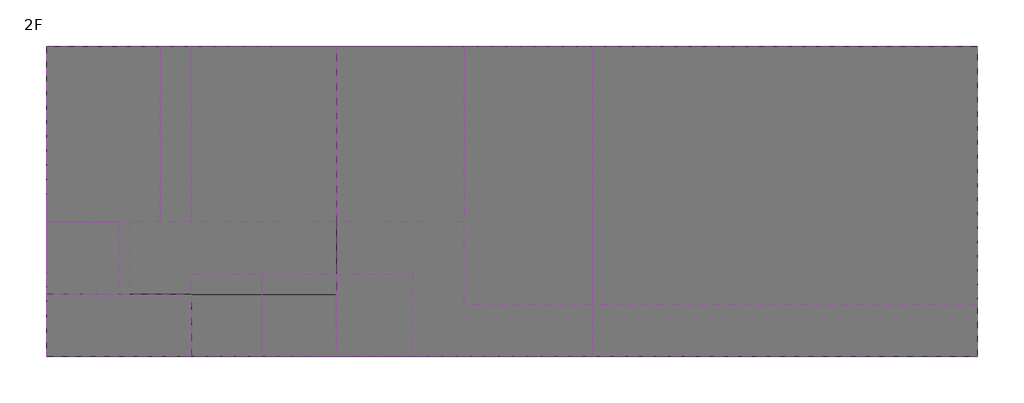
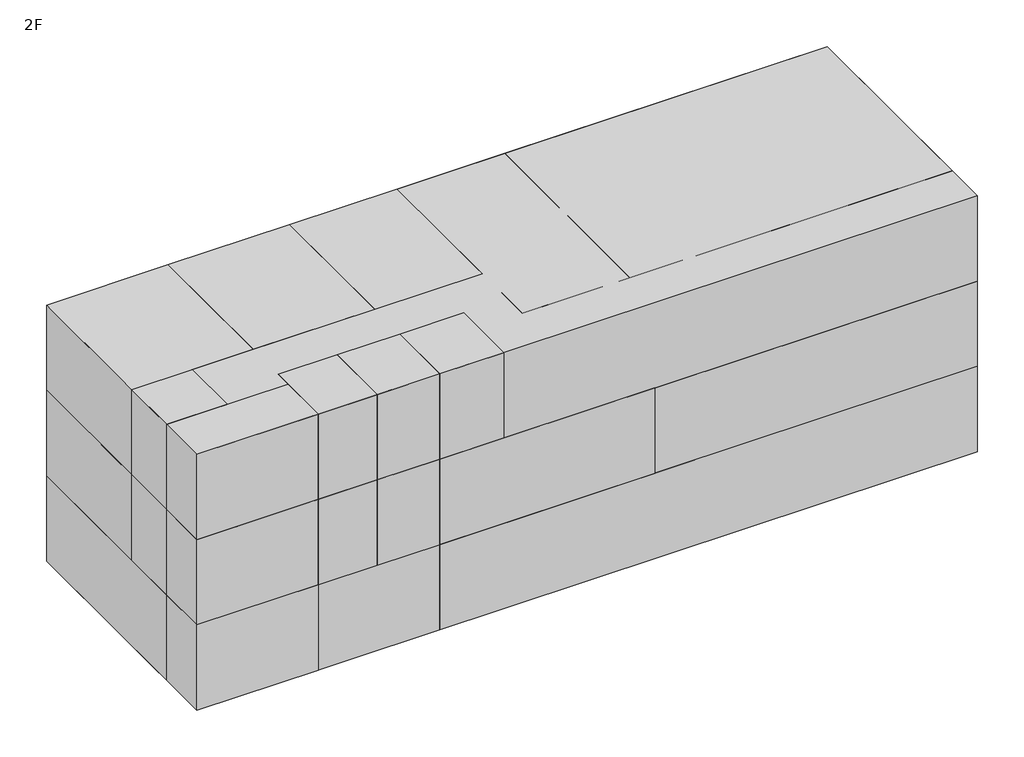
# One storey: 24 proxies.
"""IFC4 building model written with IfcOpenShell, lengths in millimetres."""

import ifcopenshell
import ifcopenshell.guid

model = None  # the IFC model being written
_history = None  # IfcOwnerHistory: only IFC2X3 demands one
_inside = {}  # id of a spatial element -> (the spatial element, [elements in it])
_under = {}  # id of a project, library or spatial element -> (it, [spatial elements below it])
_declared = {}  # id of a project -> (the project, [libraries it declares])
_typed = {}  # id of a type object -> (the type object, [elements of that type])
_made_of = {}  # id of a material, layer set ... -> (it, [elements and type objects made of it])


def new_model(schema):
    """Start an empty IFC model of exactly this schema.

    Asked for "IFC4X3", IfcOpenShell would pick the latest addendum, in which some entities
    have other attributes; the version numbers below select the first issue.
    IFC2X3 requires an IfcOwnerHistory on every rooted entity: one is made here for all.
    """
    global model, _history
    if schema == "IFC4X3":
        model = ifcopenshell.file(schema_version=(4, 3, 0, 0))
    else:
        model = ifcopenshell.file(schema=schema)
    _inside.clear()
    _under.clear()
    _declared.clear()
    _typed.clear()
    _made_of.clear()
    _history = None
    if model.schema == "IFC2X3":
        org = make("IfcOrganization", Name="unknown")
        user = make(
            "IfcPersonAndOrganization",
            ThePerson=make("IfcPerson", FamilyName="unknown"),
            TheOrganization=org,
        )
        app = make(
            "IfcApplication",
            ApplicationDeveloper=org,
            Version="unknown",
            ApplicationFullName="unknown",
            ApplicationIdentifier="unknown",
        )
        _history = make(
            "IfcOwnerHistory",
            OwningUser=user,
            OwningApplication=app,
            ChangeAction="ADDED",
            CreationDate=0,
        )
    return model


def make(cls, **values):
    """One entity of the class cls with the attributes given. An attribute that is None is left unset."""
    return model.create_entity(
        cls, **{name: value for name, value in values.items() if value is not None}
    )


def rooted(cls, **values):
    """An entity with a GlobalId (a new one), such as an element, a storey or a relation."""
    return make(cls, GlobalId=ifcopenshell.guid.new(), OwnerHistory=_history, **values)


def si_unit(unit_type, name, prefix=None):
    """IfcSIUnit, for example si_unit("LENGTHUNIT", "METRE", prefix="MILLI")."""
    return make("IfcSIUnit", UnitType=unit_type, Prefix=prefix, Name=name)


def assignment(units):
    """IfcUnitAssignment: the units of a project."""
    return None if units is None else make("IfcUnitAssignment", Units=units)


def point(xyz):
    """IfcCartesianPoint."""
    return None if xyz is None else make("IfcCartesianPoint", Coordinates=xyz)


def direction(xyz):
    """IfcDirection."""
    return None if xyz is None else make("IfcDirection", DirectionRatios=xyz)


def frame(location, z_axis=None, x_axis=None):
    """IfcAxis2Placement3D, a coordinate frame: its origin and axes. An axis left out is left unset."""
    return make(
        "IfcAxis2Placement3D",
        Location=point(location),
        Axis=direction(z_axis),
        RefDirection=direction(x_axis),
    )


def origin():
    """The frame at (0, 0, 0) with its axes left unset."""
    return frame((0.0, 0.0, 0.0))


def origin_with_axes():
    """The frame at (0, 0, 0) with the z axis (0, 0, 1) and the x axis (1, 0, 0) written out."""
    return frame((0.0, 0.0, 0.0), z_axis=(0.0, 0.0, 1.0), x_axis=(1.0, 0.0, 0.0))


def place(relative_to, where):
    """IfcLocalPlacement: puts the frame where relative to a parent placement (None: the world)."""
    return make(
        "IfcLocalPlacement", PlacementRelTo=relative_to, RelativePlacement=where
    )


def context(
    kind, dimensions, precision=None, world=None, true_north=None, identifier=None
):
    """IfcGeometricRepresentationContext, for example the 3D "Model" context."""
    return make(
        "IfcGeometricRepresentationContext",
        ContextIdentifier=identifier,
        ContextType=kind,
        CoordinateSpaceDimension=dimensions,
        Precision=precision,
        WorldCoordinateSystem=world,
        TrueNorth=true_north,
    )


def project(units=None, contexts=None):
    """IfcProject with its units and contexts."""
    return rooted(
        "IfcProject",
        Name="project",
        RepresentationContexts=contexts,
        UnitsInContext=assignment(units),
    )


def spatial(cls, under=None, at=None, **own):
    """A site, building, storey or space (cls), placed at a placement, below another one or the project."""
    s = rooted(cls, ObjectPlacement=at, **own)
    if under is not None:
        _under.setdefault(under.id(), (under, []))[1].append(s)
    return s


def polyline(points):
    """IfcPolyline through the points."""
    return make("IfcPolyline", Points=[point(p) for p in points])


def outline(outer, holes=None, kind="AREA"):
    """IfcArbitraryClosedProfileDef: a profile drawn as a closed curve; with holes, ...WithVoids."""
    if holes is None:
        return make("IfcArbitraryClosedProfileDef", ProfileType=kind, OuterCurve=outer)
    return make(
        "IfcArbitraryProfileDefWithVoids",
        ProfileType=kind,
        OuterCurve=outer,
        InnerCurves=holes,
    )


def extrude(swept, where, along, depth):
    """IfcExtrudedAreaSolid: the profile swept, set in the frame where, extruded along a direction by depth."""
    return make(
        "IfcExtrudedAreaSolid",
        SweptArea=swept,
        Position=where,
        ExtrudedDirection=direction(along),
        Depth=depth,
    )


def shape(context_of_items, identifier, shape_type, items):
    """IfcShapeRepresentation: the items that make up one representation, for example the "Body"."""
    return make(
        "IfcShapeRepresentation",
        ContextOfItems=context_of_items,
        RepresentationIdentifier=identifier,
        RepresentationType=shape_type,
        Items=items,
    )


def source(mapping_origin, context_of_items, identifier, shape_type, items):
    """IfcRepresentationMap: a shape defined once, which mapped items show again and again."""
    return make(
        "IfcRepresentationMap",
        MappingOrigin=mapping_origin,
        MappedRepresentation=shape(context_of_items, identifier, shape_type, items),
    )


def transform(
    local_origin,
    x_axis=None,
    y_axis=None,
    z_axis=None,
    scale=None,
    scale2=None,
    scale3=None,
    uniform=True,
):
    """IfcCartesianTransformationOperator3D, or its non-uniform kind. x_axis, y_axis, z_axis: its Axis1, 2, 3."""
    if uniform:
        return make(
            "IfcCartesianTransformationOperator3D",
            Axis1=direction(x_axis),
            Axis2=direction(y_axis),
            LocalOrigin=point(local_origin),
            Scale=scale,
            Axis3=direction(z_axis),
        )
    return make(
        "IfcCartesianTransformationOperator3DnonUniform",
        Axis1=direction(x_axis),
        Axis2=direction(y_axis),
        LocalOrigin=point(local_origin),
        Scale=scale,
        Axis3=direction(z_axis),
        Scale2=scale2,
        Scale3=scale3,
    )


def mapped(mapping_source, mapping_target):
    """IfcMappedItem: shows the shape of a source again, moved by a transform."""
    return make(
        "IfcMappedItem", MappingSource=mapping_source, MappingTarget=mapping_target
    )


def made_of(thing, what):
    """Note that an element or type object is made of a material, layer set ...; save() writes the relation."""
    if what is not None:
        _made_of.setdefault(what.id(), (what, []))[1].append(thing)
    return thing


def element(
    cls,
    number,
    at=None,
    inside=None,
    cuts=None,
    type_object=None,
    material=None,
    context=None,
    identifier="Body",
    shape_type=None,
    held_by="IfcProductDefinitionShape",
    body=None,
    shapes=None,
    **own,
):
    """One element of the class cls, such as IfcWall. Its Tag is "e" and its number.

    at: its placement. inside: the storey or other place that contains it. cuts: it is an
    opening in that element (IfcRelVoidsElement). A single representation is given by context,
    identifier, shape_type and body (its items); several are given by shapes. held_by: the class
    of the entity that holds the representations. save() writes the other relations.
    """
    e = rooted(cls, Tag="e%d" % number, ObjectPlacement=at, **own)
    if body is not None:
        shapes = [shape(context, identifier, shape_type, body)]
    if shapes is not None:
        e.Representation = make(held_by, Representations=shapes)
    if inside is not None:
        _inside.setdefault(inside.id(), (inside, []))[1].append(e)
    if cuts is not None:
        rooted(
            "IfcRelVoidsElement", RelatingBuildingElement=cuts, RelatedOpeningElement=e
        )
    if type_object is not None:
        _typed.setdefault(type_object.id(), (type_object, []))[1].append(e)
    return made_of(e, material)


def aggregate(whole, parts):
    """IfcRelAggregates: a whole, such as a stair, and the parts it consists of."""
    return rooted("IfcRelAggregates", RelatingObject=whole, RelatedObjects=parts)


def save(model, path):
    """Write the relations noted so far, then the file.

    IfcRelAggregates (storeys below a building ...), IfcRelContainedInSpatialStructure (elements
    in a storey), IfcRelDefinesByType, IfcRelAssociatesMaterial and IfcRelDeclares: one each for
    every whole, place, type object, material and project.
    """
    for whole, parts in _under.values():
        aggregate(whole, parts)
    for where, things in _inside.values():
        rooted(
            "IfcRelContainedInSpatialStructure",
            RelatedElements=things,
            RelatingStructure=where,
        )
    for kind, things in _typed.values():
        rooted("IfcRelDefinesByType", RelatedObjects=things, RelatingType=kind)
    for what, things in _made_of.values():
        rooted("IfcRelAssociatesMaterial", RelatedObjects=things, RelatingMaterial=what)
    for by, libraries in _declared.values():
        rooted("IfcRelDeclares", RelatingContext=by, RelatedDefinitions=libraries)
    model.write(path)


def generic_models_32ca781f(model_context):
    return source(origin(), model_context, "Body", "SweptSolid", [
        extrude(outline(polyline([(15500.0, 7500.0), (15500.0, -7500.0), (-15500.0, -7500.0), (-15500.0, 7500.0), (15500.0, 7500.0)])), origin_with_axes(), (0.0, 0.0, 1.0), 5200.0),
    ])


def generic_models_ec4f78ea(model_context):
    return source(origin(), model_context, "Body", "SweptSolid", [
        extrude(outline(polyline([(7000.0, 6000.0), (7000.0, -6000.0), (-7000.0, -6000.0), (-7000.0, 6000.0), (7000.0, 6000.0)])), origin_with_axes(), (0.0, 0.0, 1.0), 5200.0),
    ])


def generic_models_2e4aee51(model_context):
    return source(origin(), model_context, "Body", "SweptSolid", [
        extrude(outline(polyline([(1500.0, 3500.0), (1500.0, -3500.0), (-1500.0, -3500.0), (-1500.0, 3500.0), (1500.0, 3500.0)])), origin_with_axes(), (0.0, 0.0, 1.0), 5200.0),
    ])


def generic_models_246d78d5(model_context):
    return source(origin(), model_context, "Body", "SweptSolid", [
        extrude(outline(polyline([(6200.0, 7500.0), (6200.0, -7500.0), (-6200.0, -7500.0), (-6200.0, 7500.0), (6200.0, 7500.0)])), origin_with_axes(), (0.0, 0.0, 1.0), 5200.0),
    ])


def generic_models_5fb19e15(model_context):
    return source(origin(), model_context, "Body", "SweptSolid", [
        extrude(outline(polyline([(9300.0, 7500.0), (9300.0, -7500.0), (-9300.0, -7500.0), (-9300.0, 7500.0), (9300.0, 7500.0)])), origin_with_axes(), (0.0, 0.0, 1.0), 5200.0),
    ])


def generic_models_c4e3d020(model_context):
    return source(origin(), model_context, "Body", "SweptSolid", [
        extrude(outline(polyline([(4250.0, 4250.0), (4250.0, -4250.0), (-4250.0, -4250.0), (-4250.0, 4250.0), (4250.0, 4250.0)])), origin_with_axes(), (0.0, 0.0, 1.0), 5200.0),
    ])


def generic_models_d0c3260c(model_context):
    return source(origin(), model_context, "Body", "SweptSolid", [
        extrude(outline(polyline([(2750.0, 4250.0), (2750.0, -4250.0), (-2750.0, -4250.0), (-2750.0, 4250.0), (2750.0, 4250.0)])), origin_with_axes(), (0.0, 0.0, 1.0), 5200.0),
    ])


def generic_models_2b76ab57(model_context):
    return source(origin(), model_context, "Body", "SweptSolid", [
        extrude(outline(polyline([(1800.0, 2000.0), (1800.0, -2000.0), (-1800.0, -2000.0), (-1800.0, 2000.0), (1800.0, 2000.0)])), origin_with_axes(), (0.0, 0.0, 1.0), 5200.0),
    ])


def generic_models_5d679b5e(model_context):
    return source(origin(), model_context, "Body", "SweptSolid", [
        extrude(outline(polyline([(1700.0, 2000.0), (1700.0, -2000.0), (-1700.0, -2000.0), (-1700.0, 2000.0), (1700.0, 2000.0)])), origin_with_axes(), (0.0, 0.0, 1.0), 5200.0),
    ])


def generic_models_7d267c0d(model_context):
    return source(origin(), model_context, "Body", "SweptSolid", [
        extrude(outline(polyline([(1750.0, 2000.0), (1750.0, -2000.0), (-1750.0, -2000.0), (-1750.0, 2000.0), (1750.0, 2000.0)])), origin_with_axes(), (0.0, 0.0, 1.0), 5200.0),
    ])


def generic_models_235df1fa(model_context):
    return source(origin(), model_context, "Body", "SweptSolid", [
        extrude(outline(polyline([(3500.0, 4250.0), (3500.0, -4250.0), (-3500.0, -4250.0), (-3500.0, 4250.0), (3500.0, 4250.0)])), origin_with_axes(), (0.0, 0.0, 1.0), 5200.0),
    ])


def generic_models_228d8ca4(model_context):
    return source(origin(), model_context, "Body", "SweptSolid", [
        extrude(outline(polyline([(3100.0, 4250.0), (3100.0, -4250.0), (-3100.0, -4250.0), (-3100.0, 4250.0), (3100.0, 4250.0)])), origin_with_axes(), (0.0, 0.0, 1.0), 5200.0),
    ])


def generic_models_f38cfd17(model_context):
    return source(origin(), model_context, "Body", "SweptSolid", [
        extrude(outline(polyline([(3100.0, 6250.0), (3100.0, -6250.0), (-3100.0, -6250.0), (-3100.0, 6250.0), (3100.0, 6250.0)])), origin_with_axes(), (0.0, 0.0, 1.0), 5200.0),
    ])


def generic_models_0e92175d(model_context):
    return source(origin(), model_context, "Body", "SweptSolid", [
        extrude(outline(polyline([(2000.0, 1850.0), (2000.0, -1850.0), (-2000.0, -1850.0), (-2000.0, 1850.0), (2000.0, 1850.0)])), origin_with_axes(), (0.0, 0.0, 1.0), 5200.0),
    ])


def generic_models_412ad42b(model_context):
    return source(origin(), model_context, "Body", "SweptSolid", [
        extrude(outline(polyline([(1750.0, 1750.0), (1750.0, -1750.0), (-1750.0, -1750.0), (-1750.0, 1750.0), (1750.0, 1750.0)])), origin_with_axes(), (0.0, 0.0, 1.0), 5200.0),
    ])


def generic_models_608d95d2(model_context):
    return source(origin(), model_context, "Body", "SweptSolid", [
        extrude(outline(polyline([(9300.0, 6250.0), (9300.0, -6250.0), (-9300.0, -6250.0), (-9300.0, 6250.0), (9300.0, 6250.0)])), origin_with_axes(), (0.0, 0.0, 1.0), 5200.0),
    ])


def generic_models_083cc7c1(model_context):
    return source(origin(), model_context, "Body", "SweptSolid", [
        extrude(outline(polyline([(7500.0, 22500.0), (7500.0, -22500.0), (-7500.0, -22500.0), (-7500.0, 22500.0), (7500.0, 22500.0)])), origin_with_axes(), (0.0, 0.0, 1.0), 5200.0),
    ])


model = new_model("IFC4")

# Units and contexts
model_context = context("Model", 3, world=origin())
ifc_project = project(units=[si_unit("LENGTHUNIT", "METRE", prefix="MILLI")], contexts=[model_context])

# Site, building, storey
site = spatial("IfcSite", under=ifc_project)
building = spatial("IfcBuilding", under=site)
storey = spatial("IfcBuildingStorey", under=building, Name="2F", Elevation=5500.0)

# Proxies
placement = place(None, origin())
generic_models_shape = generic_models_32ca781f(model_context)
element("IfcBuildingElementProxy", 1, Name="Space Planning Box_hec : Space Planning Box_hec", ObjectType="Space Planning Box_hec : Space Planning Box_hec", at=placement, inside=storey, context=model_context, shape_type="MappedRepresentation", body=[
    mapped(generic_models_shape, transform((74959.6521483, 179923.8614395, 5500.0), x_axis=(1.0, 0.0, 0.0), y_axis=(0.0, 1.0, 0.0), z_axis=(0.0, 0.0, 1.0))),
])
generic_models_2_shape = generic_models_ec4f78ea(model_context)
element("IfcBuildingElementProxy", 2, Name="Space Planning Box_hec : Space Planning Box_hec", ObjectType="Space Planning Box_hec : Space Planning Box_hec", at=placement, inside=storey, context=model_context, shape_type="MappedRepresentation", body=[
    mapped(generic_models_2_shape, transform((52459.6521483, 181423.8614395, 5500.0), x_axis=(1.0, 0.0, 0.0), y_axis=(0.0, 1.0, 0.0), z_axis=(0.0, 0.0, 1.0))),
])
generic_models_3_shape = generic_models_2e4aee51(model_context)
element("IfcBuildingElementProxy", 3, Name="Space Planning Box_hec : Space Planning Box_hec", ObjectType="Space Planning Box_hec : Space Planning Box_hec", at=placement, inside=storey, context=model_context, shape_type="MappedRepresentation", body=[
    mapped(generic_models_3_shape, transform((48959.6521483, 173923.8614395, 5500.0), x_axis=(0.0, 1.0, 0.0), y_axis=(-1.0, 0.0, 0.0), z_axis=(0.0, 0.0, 1.0))),
])
element("IfcBuildingElementProxy", 4, Name="Space Planning Box_hec : Space Planning Box_hec", ObjectType="Space Planning Box_hec : Space Planning Box_hec", at=placement, inside=storey, context=model_context, shape_type="MappedRepresentation", body=[
    mapped(generic_models_3_shape, transform((48959.6521483, 173923.8614395, 10700.0), x_axis=(0.0, 1.0, 0.0), y_axis=(-1.0, 0.0, 0.0), z_axis=(0.0, 0.0, 1.0))),
])
element("IfcBuildingElementProxy", 5, Name="Space Planning Box_hec : Space Planning Box_hec", ObjectType="Space Planning Box_hec : Space Planning Box_hec", at=placement, inside=storey, context=model_context, shape_type="MappedRepresentation", body=[
    mapped(generic_models_3_shape, transform((48959.6521483, 173923.8614395, 15900.0), x_axis=(0.0, 1.0, 0.0), y_axis=(-1.0, 0.0, 0.0), z_axis=(0.0, 0.0, 1.0))),
])
generic_models_4_shape = generic_models_246d78d5(model_context)
element("IfcBuildingElementProxy", 6, Name="Space Planning Box_hec : Space Planning Box_hec", ObjectType="Space Planning Box_hec : Space Planning Box_hec", at=placement, inside=storey, context=model_context, shape_type="MappedRepresentation", body=[
    mapped(generic_models_4_shape, transform((65659.6521483, 179923.8614395, 10700.0), x_axis=(1.0, 0.0, 0.0), y_axis=(0.0, 1.0, 0.0), z_axis=(0.0, 0.0, 1.0))),
])
generic_models_5_shape = generic_models_5fb19e15(model_context)
element("IfcBuildingElementProxy", 7, Name="Space Planning Box_hec : Space Planning Box_hec", ObjectType="Space Planning Box_hec : Space Planning Box_hec", at=placement, inside=storey, context=model_context, shape_type="MappedRepresentation", body=[
    mapped(generic_models_5_shape, transform((81159.6521483, 179923.8614395, 10700.0), x_axis=(1.0, 0.0, 0.0), y_axis=(0.0, 1.0, 0.0), z_axis=(0.0, 0.0, 1.0))),
])
generic_models_6_shape = generic_models_c4e3d020(model_context)
element("IfcBuildingElementProxy", 8, Name="Space Planning Box_hec : Space Planning Box_hec", ObjectType="Space Planning Box_hec : Space Planning Box_hec", at=placement, inside=storey, context=model_context, shape_type="MappedRepresentation", body=[
    mapped(generic_models_6_shape, transform((55209.6521483, 183173.8614395, 10700.0), x_axis=(-1.0, 0.0, 0.0), y_axis=(0.0, -1.0, 0.0), z_axis=(0.0, 0.0, 1.0))),
])
generic_models_7_shape = generic_models_d0c3260c(model_context)
element("IfcBuildingElementProxy", 9, Name="Space Planning Box_hec : Space Planning Box_hec", ObjectType="Space Planning Box_hec : Space Planning Box_hec", at=placement, inside=storey, context=model_context, shape_type="MappedRepresentation", body=[
    mapped(generic_models_7_shape, transform((48209.6521483, 183173.8614395, 10700.0), x_axis=(1.0, 0.0, 0.0), y_axis=(0.0, 1.0, 0.0), z_axis=(0.0, 0.0, 1.0))),
])
generic_models_8_shape = generic_models_2b76ab57(model_context)
element("IfcBuildingElementProxy", 10, Name="Space Planning Box_hec : Space Planning Box_hec", ObjectType="Space Planning Box_hec : Space Planning Box_hec", at=placement, inside=storey, context=model_context, shape_type="MappedRepresentation", body=[
    mapped(generic_models_8_shape, transform((57659.6521483, 174423.8614395, 10700.0), x_axis=(1.0, 0.0, 0.0), y_axis=(0.0, 1.0, 0.0), z_axis=(0.0, 0.0, 1.0))),
])
element("IfcBuildingElementProxy", 11, Name="Space Planning Box_hec : Space Planning Box_hec", ObjectType="Space Planning Box_hec : Space Planning Box_hec", at=placement, inside=storey, context=model_context, shape_type="MappedRepresentation", body=[
    mapped(generic_models_8_shape, transform((57659.6521483, 174423.8614395, 15900.0), x_axis=(1.0, 0.0, 0.0), y_axis=(0.0, 1.0, 0.0), z_axis=(0.0, 0.0, 1.0))),
])
generic_models_9_shape = generic_models_5d679b5e(model_context)
element("IfcBuildingElementProxy", 12, Name="Space Planning Box_hec : Space Planning Box_hec", ObjectType="Space Planning Box_hec : Space Planning Box_hec", at=placement, inside=storey, context=model_context, shape_type="MappedRepresentation", body=[
    mapped(generic_models_9_shape, transform((54159.6521483, 174423.8614395, 10700.0), x_axis=(1.0, 0.0, 0.0), y_axis=(0.0, 1.0, 0.0), z_axis=(0.0, 0.0, 1.0))),
])
element("IfcBuildingElementProxy", 13, Name="Space Planning Box_hec : Space Planning Box_hec", ObjectType="Space Planning Box_hec : Space Planning Box_hec", at=placement, inside=storey, context=model_context, shape_type="MappedRepresentation", body=[
    mapped(generic_models_9_shape, transform((54159.6521483, 174423.8614395, 15900.0), x_axis=(1.0, 0.0, 0.0), y_axis=(0.0, 1.0, 0.0), z_axis=(0.0, 0.0, 1.0))),
])
generic_models_10_shape = generic_models_7d267c0d(model_context)
element("IfcBuildingElementProxy", 14, Name="Space Planning Box_hec : Space Planning Box_hec", ObjectType="Space Planning Box_hec : Space Planning Box_hec", at=placement, inside=storey, context=model_context, shape_type="MappedRepresentation", body=[
    mapped(generic_models_10_shape, transform((47459.6521483, 177173.8614395, 10700.0), x_axis=(0.0, 1.0, 0.0), y_axis=(-1.0, 0.0, 0.0), z_axis=(0.0, 0.0, 1.0))),
])
generic_models_11_shape = generic_models_235df1fa(model_context)
element("IfcBuildingElementProxy", 15, Name="Space Planning Box_hec : Space Planning Box_hec", ObjectType="Space Planning Box_hec : Space Planning Box_hec", at=placement, inside=storey, context=model_context, shape_type="MappedRepresentation", body=[
    mapped(generic_models_11_shape, transform((48959.6521483, 183173.8614395, 15900.0), x_axis=(1.0, 0.0, 0.0), y_axis=(0.0, 1.0, 0.0), z_axis=(0.0, 0.0, 1.0))),
])
element("IfcBuildingElementProxy", 16, Name="Space Planning Box_hec : Space Planning Box_hec", ObjectType="Space Planning Box_hec : Space Planning Box_hec", at=placement, inside=storey, context=model_context, shape_type="MappedRepresentation", body=[
    mapped(generic_models_11_shape, transform((55959.6521483, 183173.8614395, 15900.0), x_axis=(-1.0, 0.0, 0.0), y_axis=(0.0, -1.0, 0.0), z_axis=(0.0, 0.0, 1.0))),
])
generic_models_12_shape = generic_models_228d8ca4(model_context)
element("IfcBuildingElementProxy", 17, Name="Space Planning Box_hec : Space Planning Box_hec", ObjectType="Space Planning Box_hec : Space Planning Box_hec", at=placement, inside=storey, context=model_context, shape_type="MappedRepresentation", body=[
    mapped(generic_models_12_shape, transform((62559.6521483, 183173.8614395, 15900.0), x_axis=(1.0, 0.0, 0.0), y_axis=(0.0, 1.0, 0.0), z_axis=(0.0, 0.0, 1.0))),
])
generic_models_13_shape = generic_models_f38cfd17(model_context)
element("IfcBuildingElementProxy", 18, Name="Space Planning Box_hec : Space Planning Box_hec", ObjectType="Space Planning Box_hec : Space Planning Box_hec", at=placement, inside=storey, context=model_context, shape_type="MappedRepresentation", body=[
    mapped(generic_models_13_shape, transform((68759.6521483, 181173.8614395, 15900.0), x_axis=(1.0, 0.0, 0.0), y_axis=(0.0, 1.0, 0.0), z_axis=(0.0, 0.0, 1.0))),
])
generic_models_14_shape = generic_models_0e92175d(model_context)
element("IfcBuildingElementProxy", 19, Name="Space Planning Box_hec : Space Planning Box_hec", ObjectType="Space Planning Box_hec : Space Planning Box_hec", at=placement, inside=storey, context=model_context, shape_type="MappedRepresentation", body=[
    mapped(generic_models_14_shape, transform((61309.6521483, 174423.8614395, 15900.0), x_axis=(0.0, 1.0, 0.0), y_axis=(-1.0, 0.0, 0.0), z_axis=(0.0, 0.0, 1.0))),
])
generic_models_15_shape = generic_models_412ad42b(model_context)
element("IfcBuildingElementProxy", 20, Name="Space Planning Box_hec : Space Planning Box_hec", ObjectType="Space Planning Box_hec : Space Planning Box_hec", at=placement, inside=storey, context=model_context, shape_type="MappedRepresentation", body=[
    mapped(generic_models_15_shape, transform((47209.6521483, 177173.8614395, 15900.0), x_axis=(1.0, 0.0, 0.0), y_axis=(0.0, 1.0, 0.0), z_axis=(0.0, 0.0, 1.0))),
])
generic_models_16_shape = generic_models_608d95d2(model_context)
element("IfcBuildingElementProxy", 21, Name="Space Planning Box_hec : Space Planning Box_hec", ObjectType="Space Planning Box_hec : Space Planning Box_hec", at=placement, inside=storey, context=model_context, shape_type="MappedRepresentation", body=[
    mapped(generic_models_16_shape, transform((81159.6521483, 181173.8614395, 15900.0), x_axis=(1.0, 0.0, 0.0), y_axis=(0.0, 1.0, 0.0), z_axis=(0.0, 0.0, 1.0))),
])
generic_models_17_shape = generic_models_083cc7c1(model_context)
element("IfcBuildingElementProxy", 22, Name="Space Planning Box_hec : Space Planning Box_hec", ObjectType="Space Planning Box_hec : Space Planning Box_hec", at=placement, inside=storey, context=model_context, shape_type="MappedRepresentation", body=[
    mapped(generic_models_17_shape, transform((67959.6521483, 179923.8614395, 5500.0), x_axis=(0.0, 1.0, 0.0), y_axis=(-1.0, 0.0, 0.0), z_axis=(0.0, 0.0, 1.0))),
])
element("IfcBuildingElementProxy", 23, Name="Space Planning Box_hec : Space Planning Box_hec", ObjectType="Space Planning Box_hec : Space Planning Box_hec", at=placement, inside=storey, context=model_context, shape_type="MappedRepresentation", body=[
    mapped(generic_models_17_shape, transform((67959.6521483, 179923.8614395, 10700.0), x_axis=(0.0, 1.0, 0.0), y_axis=(-1.0, 0.0, 0.0), z_axis=(0.0, 0.0, 1.0))),
])
element("IfcBuildingElementProxy", 24, Name="Space Planning Box_hec : Space Planning Box_hec", ObjectType="Space Planning Box_hec : Space Planning Box_hec", at=placement, inside=storey, context=model_context, shape_type="MappedRepresentation", body=[
    mapped(generic_models_17_shape, transform((67959.6521483, 179923.8614395, 15900.0), x_axis=(0.0, -1.0, 0.0), y_axis=(1.0, 0.0, 0.0), z_axis=(0.0, 0.0, 1.0))),
])

save(model, "model.ifc")

# Revit data of these elements
# Project information
#   Building Name = "MAIN GATE SECURITY BUILDING"
#   Project Status = "Project Status"
#   Client Name = "현대엔지니어링"
#   Project Address = "서울시 종로구 율곡로 75(계동)"
#   Project Name = "Therma Visayas Energy Project"
#   Project Number = "-"
# Grids (mm)
#   "1": line (459.652, 194613.421) -> (459.652, 156518.279)
#   "2": line (7459.652, 194613.421) -> (7459.652, 156518.279)
#   "3": line (14459.652, 194613.421) -> (14459.652, 156518.279)
#   "4": line (20659.652, 194613.421) -> (20659.652, 156518.279)
#   "5": line (26859.652, 194613.421) -> (26859.652, 156518.279)
#   "6": line (33059.652, 194613.421) -> (33059.652, 156518.279)
#   "7": line (39259.652, 194613.421) -> (39259.652, 156518.279)
#   "8": line (45459.652, 194613.421) -> (45459.652, 156518.279)
#   "C": line (39389.066, 187423.861) -> (102402.798, 187423.861)
#   "B": line (39389.066, 178923.861) -> (102402.798, 178923.861)
#   "A": line (39389.066, 172423.861) -> (102402.798, 172423.861)
# Type "Space Planning Box_hec : Space Planning Box_hec"
#   Type Comments = "..."
#   Room Name [instance default] = "?"
#   Interior Finish [instance default] = ""
#   Exterior Finish [instance default] = ""
#   Department [instance default] = ""
#   Assembly Code = "..."
#   ceiling height [instance default] = 0
#   Width [instance default] = 1524 mm
#   Program Area [instance default] = 0.00 m²
#   Length [instance default] = 1524 mm
#   Height [instance default] = 1524 mm
#   Area [instance default] = 2.32258 m²
#   Fill Color [instance default] = Cyan
#   Default Elevation = 0
# Element 1 (IfcBuildingElementProxy, "Space Planning Box_hec : Space Planning Box_hec")
#   Room Name = "Electrical Room"
#   Interior Finish = "IW1..N/A,,WB1..N/A,,FL2..N/A,,CL1..N/A"
#   Exterior Finish = "N/A..N/A,,EW1..N/A"
#   Department = "EL"
#   ceiling height = 0
#   Width = 31000 mm
#   Program Area = 465.00 m²
#   Length = 15000 mm
#   Height = 5200 mm
#   Area = 465.00 m²
#   Fill Color = Orange
#   Phase Created = New Construction
#   Materials on its faces: "Orange"
# Element 2 (IfcBuildingElementProxy, "Space Planning Box_hec : Space Planning Box_hec")
#   Room Name = "Battery Room"
#   Interior Finish = "IW2..N/A,,WB4..N/A,,FL3..N/A,,CL2..N/A"
#   Exterior Finish = "N/A..N/A,,EW1..N/A"
#   Department = "EL"
#   ceiling height = 0
#   Width = 14000 mm
#   Program Area = 168.00 m²
#   Length = 12000 mm
#   Height = 5200 mm
#   Area = 168.00 m²
#   Fill Color = Orange
#   Phase Created = New Construction
#   Materials on its faces: "Orange"
# Elements 3, 4 (IfcBuildingElementProxy, "Space Planning Box_hec : Space Planning Box_hec")
#   Room Name = "Staircase"
#   Interior Finish = "IW1..N/A,,WB2..N/A,,FL6..N/A,,CL1..N/A"
#   Exterior Finish = "N/A..N/A,,EW1..N/A"
#   Department = "AR"
#   ceiling height = 0
#   Width = 3000 mm
#   Program Area = 21.00 m²
#   Length = 7000 mm
#   Height = 5200 mm
#   Area = 21.00 m²
#   Fill Color = Cyan
#   Phase Created = New Construction
#   Materials on its faces: "Cyan"
# Element 5 (IfcBuildingElementProxy, "Space Planning Box_hec : Space Planning Box_hec")
#   Room Name = "Staircase"
#   Interior Finish = "IW1..N/A,,WB2..N/A,,FL6..N/A,,CL1..N/A"
#   Exterior Finish = "RF1..N/A,,EW1..N/A"
#   Department = "AR"
#   ceiling height = 0
#   Width = 3000 mm
#   Program Area = 21.00 m²
#   Length = 7000 mm
#   Height = 5200 mm
#   Area = 21.00 m²
#   Fill Color = Cyan
#   Phase Created = New Construction
#   Materials on its faces: "Cyan"
# Element 6 (IfcBuildingElementProxy, "Space Planning Box_hec : Space Planning Box_hec")
#   Room Name = "Central Control Room"
#   Interior Finish = "IW1..N/A,,WB2..N/A,,FL7..N/A,,CL4..N/A"
#   Exterior Finish = "N/A..N/A,,EW1..N/A"
#   Department = "CI"
#   ceiling height = 3400
#   Width = 12400 mm
#   Program Area = 186.00 m²
#   Length = 15000 mm
#   Height = 5200 mm
#   Area = 186.00 m²
#   Fill Color = Yellow
#   Phase Created = New Construction
#   Materials on its faces: "Yellow"
# Element 7 (IfcBuildingElementProxy, "Space Planning Box_hec : Space Planning Box_hec")
#   Room Name = "Electronic Room"
#   Interior Finish = "IW1..N/A,,WB2..N/A,,FL7..N/A,,CL4..N/A"
#   Exterior Finish = "N/A..N/A,,EW1..N/A"
#   Department = "CI"
#   ceiling height = 3000
#   Width = 18600 mm
#   Program Area = 279.00 m²
#   Length = 15000 mm
#   Height = 5200 mm
#   Area = 279.00 m²
#   Fill Color = Yellow
#   Phase Created = New Construction
#   Materials on its faces: "Yellow"
# Element 8 (IfcBuildingElementProxy, "Space Planning Box_hec : Space Planning Box_hec")
#   Room Name = "Computer Room"
#   Interior Finish = "IW1..N/A,,WB2..N/A,,FL7..N/A,,CL4..N/A"
#   Exterior Finish = "N/A..N/A,,EW1..N/A"
#   Department = "CI"
#   ceiling height = 2700
#   Width = 8500 mm
#   Program Area = 72.25 m²
#   Length = 8500 mm
#   Height = 5200 mm
#   Area = 72.25 m²
#   Fill Color = Yellow
#   Phase Created = New Construction
#   Materials on its faces: "Yellow"
# Element 9 (IfcBuildingElementProxy, "Space Planning Box_hec : Space Planning Box_hec")
#   Room Name = "Communication Room"
#   Interior Finish = "IW1..N/A,,WB2..N/A,,FL7..N/A,,CL4..N/A"
#   Exterior Finish = "N/A..N/A,,EW1..N/A"
#   Department = "CI"
#   ceiling height = 2700
#   Width = 5500 mm
#   Program Area = 46.75 m²
#   Length = 8500 mm
#   Height = 5200 mm
#   Area = 46.75 m²
#   Fill Color = Yellow
#   Phase Created = New Construction
#   Materials on its faces: "Yellow"
# Element 10 (IfcBuildingElementProxy, "Space Planning Box_hec : Space Planning Box_hec")
#   Room Name = "Toilet (M)"
#   Interior Finish = "IW3..N/A,,N/A..N/A,,FL5..N/A,,CL5..N/A"
#   Exterior Finish = "N/A..N/A,,EW1..N/A"
#   Department = "AR"
#   ceiling height = 2400
#   Width = 3600 mm
#   Program Area = 14.40 m²
#   Length = 4000 mm
#   Height = 5200 mm
#   Area = 14.40 m²
#   Fill Color = Cyan
#   Phase Created = New Construction
#   Materials on its faces: "Cyan"
# Element 11 (IfcBuildingElementProxy, "Space Planning Box_hec : Space Planning Box_hec")
#   Room Name = "Toilet (M)"
#   Interior Finish = "IW3..N/A,,N/A..N/A,,FL5..N/A,,CL5..N/A"
#   Exterior Finish = "RF1..N/A,,EW1..N/A"
#   Department = "AR"
#   ceiling height = 2400
#   Width = 3600 mm
#   Program Area = 14.40 m²
#   Length = 4000 mm
#   Height = 5200 mm
#   Area = 14.40 m²
#   Fill Color = Cyan
#   Phase Created = New Construction
#   Materials on its faces: "Cyan"
# Element 12 (IfcBuildingElementProxy, "Space Planning Box_hec : Space Planning Box_hec")
#   Room Name = "Toilet(F)"
#   Interior Finish = "IW3..N/A,,N/A..N/A,,FL5..N/A,,CL5..N/A"
#   Exterior Finish = "N/A..N/A,,EW1..N/A"
#   Department = "AR"
#   ceiling height = 2400
#   Width = 3400 mm
#   Program Area = 13.60 m²
#   Length = 4000 mm
#   Height = 5200 mm
#   Area = 13.60 m²
#   Fill Color = Cyan
#   Phase Created = New Construction
#   Materials on its faces: "Cyan"
# Element 13 (IfcBuildingElementProxy, "Space Planning Box_hec : Space Planning Box_hec")
#   Room Name = "Toilet(F)"
#   Interior Finish = "IW3..N/A,,N/A..N/A,,FL5..N/A,,CL5..N/A"
#   Exterior Finish = "RF1..N/A,,EW1..N/A"
#   Department = "AR"
#   ceiling height = 2400
#   Width = 3400 mm
#   Program Area = 13.60 m²
#   Length = 4000 mm
#   Height = 5200 mm
#   Area = 13.60 m²
#   Fill Color = Cyan
#   Phase Created = New Construction
#   Materials on its faces: "Cyan"
# Element 14 (IfcBuildingElementProxy, "Space Planning Box_hec : Space Planning Box_hec")
#   Room Name = "Pantry"
#   Interior Finish = "IW1..N/A,,WB2..N/A,,FL6..N/A,,CL4..N/A"
#   Exterior Finish = "RF1..N/A,,EW1..N/A"
#   Department = "AR"
#   ceiling height = 2700
#   Width = 3500 mm
#   Program Area = 14.00 m²
#   Length = 4000 mm
#   Height = 5200 mm
#   Area = 14.00 m²
#   Fill Color = Cyan
#   Phase Created = New Construction
#   Materials on its faces: "Cyan"
# Element 15 (IfcBuildingElementProxy, "Space Planning Box_hec : Space Planning Box_hec")
#   Room Name = "Office-1"
#   Interior Finish = "IW1..N/A,,WB2..N/A,,FL6..N/A,,CL4..N/A"
#   Exterior Finish = "RF1..N/A,,EW1..N/A"
#   Department = "AR"
#   ceiling height = 2700
#   Width = 7000 mm
#   Program Area = 59.50 m²
#   Length = 8500 mm
#   Height = 5200 mm
#   Area = 59.50 m²
#   Fill Color = Cyan
#   Phase Created = New Construction
#   Materials on its faces: "Cyan"
# Element 16 (IfcBuildingElementProxy, "Space Planning Box_hec : Space Planning Box_hec")
#   Room Name = "Office-2"
#   Interior Finish = "IW1..N/A,,WB2..N/A,,FL6..N/A,,CL4..N/A"
#   Exterior Finish = "RF1..N/A,,EW1..N/A"
#   Department = "AR"
#   ceiling height = 2700
#   Width = 7000 mm
#   Program Area = 59.50 m²
#   Length = 8500 mm
#   Height = 5200 mm
#   Area = 59.50 m²
#   Fill Color = Cyan
#   Phase Created = New Construction
#   Materials on its faces: "Cyan"
# Element 17 (IfcBuildingElementProxy, "Space Planning Box_hec : Space Planning Box_hec")
#   Room Name = "Meeting Room-1"
#   Interior Finish = "IW1..N/A,,WB2..N/A,,FL6..N/A,,CL4..N/A"
#   Exterior Finish = "RF1..N/A,,EW1..N/A"
#   Department = "AR"
#   ceiling height = 2700
#   Width = 6200 mm
#   Program Area = 52.70 m²
#   Length = 8500 mm
#   Height = 5200 mm
#   Area = 52.70 m²
#   Fill Color = Cyan
#   Phase Created = New Construction
#   Materials on its faces: "Cyan"
# Element 18 (IfcBuildingElementProxy, "Space Planning Box_hec : Space Planning Box_hec")
#   Room Name = "Office-3"
#   Interior Finish = "IW1..N/A,,WB2..N/A,,FL6..N/A,,CL4..N/A"
#   Exterior Finish = "RF1..N/A,,EW1..N/A"
#   Department = "AR"
#   ceiling height = 2700
#   Width = 6200 mm
#   Program Area = 77.50 m²
#   Length = 12500 mm
#   Height = 5200 mm
#   Area = 77.50 m²
#   Fill Color = Cyan
#   Phase Created = New Construction
#   Materials on its faces: "Cyan"
# Element 19 (IfcBuildingElementProxy, "Space Planning Box_hec : Space Planning Box_hec")
#   Room Name = "Pantry"
#   Interior Finish = "IW1..N/A,,WB2..N/A,,FL6..N/A,,CL4..N/A"
#   Exterior Finish = "RF1..N/A,,EW1..N/A"
#   Department = "AR"
#   ceiling height = 2700
#   Width = 4000 mm
#   Program Area = 14.80 m²
#   Length = 3700 mm
#   Height = 5200 mm
#   Area = 14.80 m²
#   Fill Color = Cyan
#   Phase Created = New Construction
#   Materials on its faces: "Cyan"
# Element 20 (IfcBuildingElementProxy, "Space Planning Box_hec : Space Planning Box_hec")
#   Room Name = "Storage"
#   Interior Finish = "IW1..N/A,,WB2..N/A,,FL2..N/A,,CL4..N/A"
#   Exterior Finish = "RF1..N/A,,EW1..N/A"
#   Department = "AR"
#   ceiling height = 2700
#   Width = 3500 mm
#   Program Area = 12.25 m²
#   Length = 3500 mm
#   Height = 5200 mm
#   Area = 12.25 m²
#   Fill Color = Cyan
#   Phase Created = New Construction
#   Materials on its faces: "Cyan"
# Element 21 (IfcBuildingElementProxy, "Space Planning Box_hec : Space Planning Box_hec")
#   Room Name = "HVAC Room"
#   Interior Finish = "IW1..N/A,,WB1..N/A,,FL2..N/A,,CL1..N/A"
#   Exterior Finish = "RF1..N/A,,EW1..N/A"
#   Department = "HV"
#   ceiling height = 0
#   Width = 18600 mm
#   Program Area = 232.50 m²
#   Length = 12500 mm
#   Height = 5200 mm
#   Area = 232.50 m²
#   Fill Color = Lime
#   Phase Created = New Construction
#   Materials on its faces: "Lime"
# Element 22 (IfcBuildingElementProxy, "Space Planning Box_hec : Space Planning Box_hec")
#   Room Name = "Corridor"
#   Interior Finish = "IW1..N/A,,WB2..N/A,,FL6..N/A,,CL4..N/A"
#   Exterior Finish = "N/A..N/A,,EW1..N/A"
#   Department = "AR"
#   ceiling height = 2700
#   Width = 15000 mm
#   Program Area = 21.00 m²
#   Length = 45000 mm
#   Height = 5200 mm
#   Area = 675.00 m²
#   Fill Color = Cyan
#   Phase Created = New Construction
#   Materials on its faces: "Cyan"
# Element 23 (IfcBuildingElementProxy, "Space Planning Box_hec : Space Planning Box_hec")
#   Room Name = "Corridor"
#   Interior Finish = "IW1..N/A,,WB2..N/A,,FL6..N/A,,CL4..N/A"
#   Exterior Finish = "N/A..N/A,,EW1..N/A"
#   Department = "AR"
#   ceiling height = 2700
#   Width = 15000 mm
#   Program Area = 28.00 m²
#   Length = 45000 mm
#   Height = 5200 mm
#   Area = 675.00 m²
#   Fill Color = Cyan
#   Phase Created = New Construction
#   Materials on its faces: "Cyan"
# Element 24 (IfcBuildingElementProxy, "Space Planning Box_hec : Space Planning Box_hec")
#   Room Name = "Corridor"
#   Interior Finish = "IW1..N/A,,WB2..N/A,,FL6..N/A,,CL4..N/A"
#   Exterior Finish = "RF1..N/A,,EW1..N/A"
#   Department = "AR"
#   ceiling height = 2700
#   Width = 15000 mm
#   Program Area = 117.25 m²
#   Length = 45000 mm
#   Height = 5200 mm
#   Area = 675.00 m²
#   Fill Color = Cyan
#   Phase Created = New Construction
#   Materials on its faces: "Cyan"
# Materials
#   "Cyan": class "Generic", colour RGB 0 255 255, transparency 0.2, Cost = 0
#   "Orange": class "Generic", colour RGB 255 165 0, transparency 0.2, Cost = 0
#   "Yellow": class "Generic", colour RGB 255 255 0, transparency 0.2, Cost = 0
#   "Lime": class "Generic", colour RGB 0 255 0, transparency 0.2, Cost = 0
